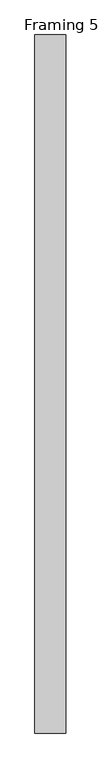
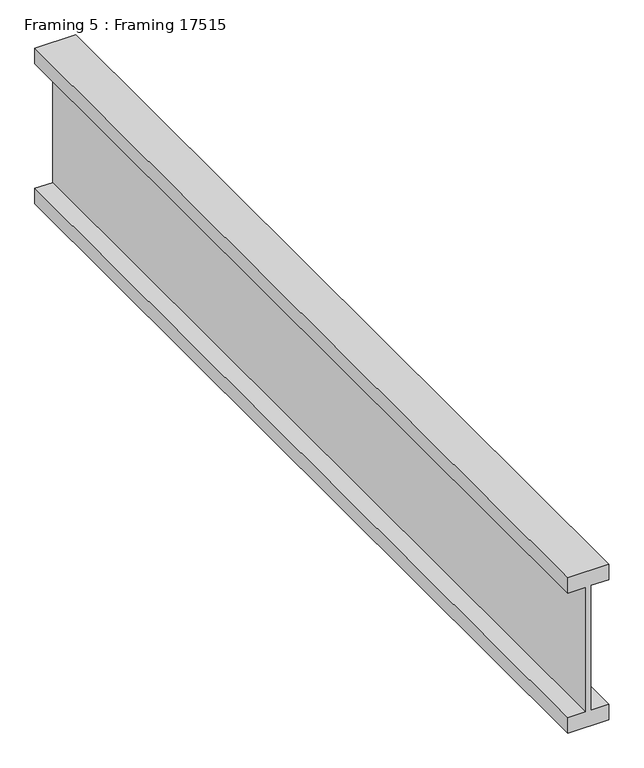
"""IFC4 building model written with IfcOpenShell, lengths in millimetres: proxy geometry, Framing 5 : Framing 17515."""

from ifc_helpers import new_model, si_unit, frame, origin, place, context, project, spatial, polyline, outline, extrude, source, transform, mapped, element, save


def framing_5_framing_17515_e96781f7(model_context):
    return source(origin(), model_context, "Body", "SweptSolid", [
        extrude(outline(polyline([(40077.771, 7689.895938), (39792.021, 7689.895938), (39792.021, 7651.002188), (39757.096, 7651.002188), (39757.096, 7739.902188), (39792.021, 7739.902188), (39792.021, 7701.008438), (40077.771, 7701.008438), (40077.771, 7739.902188), (40112.696, 7739.902188), (40112.696, 7651.002188), (40077.771, 7651.002188), (40077.771, 7689.895938)])), frame((0.0, -3747.9491938, 0.0), z_axis=(0.0, 1.0, 0.0), x_axis=(0.0, 0.0, 1.0)), (0.0, 0.0, 1.0), 2000.0),
    ])


if __name__ == "__main__":
    model = new_model("IFC4")
    model_context = context("Model", 3, world=origin())
    ifc_project = project(units=[si_unit("LENGTHUNIT", "METRE", prefix="MILLI")], contexts=[model_context])
    site = spatial("IfcSite", under=ifc_project)
    building = spatial("IfcBuilding", under=site)
    placement = place(None, origin())
    framing_5_framing_17515_shape = framing_5_framing_17515_e96781f7(model_context)
    element("IfcBuildingElementProxy", 1, Name="Framing 5 : Framing 17515", ObjectType="Framing 5 : Framing 17515", at=placement, inside=building, context=model_context, shape_type="MappedRepresentation", body=[
        mapped(framing_5_framing_17515_shape, transform((0.0, 0.0, 0.0), x_axis=(1.0, 0.0, 0.0), y_axis=(0.0, 1.0, 0.0), z_axis=(0.0, 0.0, 1.0))),
    ])
    save(model, "model.ifc")

# Revit data of these elements
# Type "Framing 5 : Framing 17515"
#   NameOverride = "Framing"
# Element 1 (IfcBuildingElementProxy, "Framing 5 : Framing 17515")
#   Materials on its faces: "WOOD FRAMING (SEE STRUCT DWGS)"
# Materials
#   "WOOD FRAMING (SEE STRUCT DWGS)": class "Unassigned", colour RGB 224 188 168, transparency 0, Cost = 0
